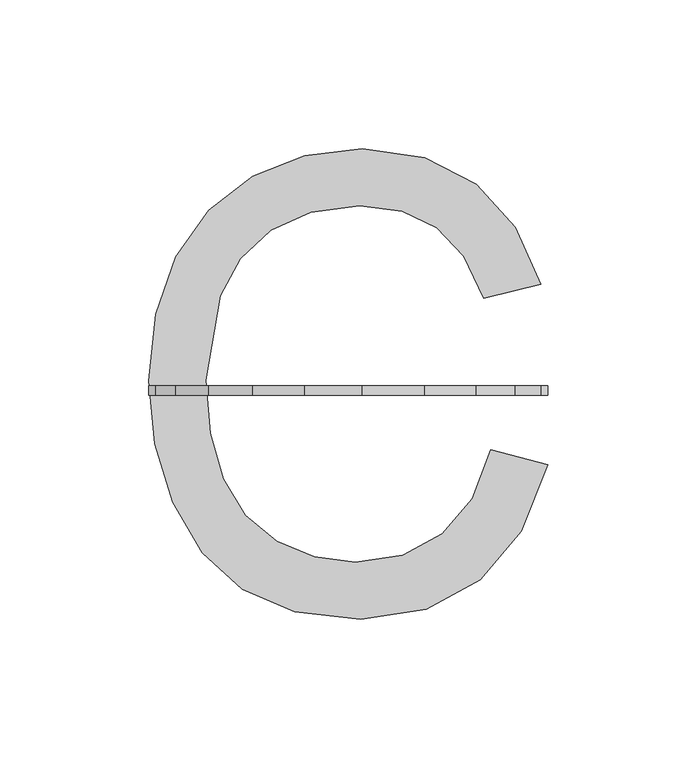
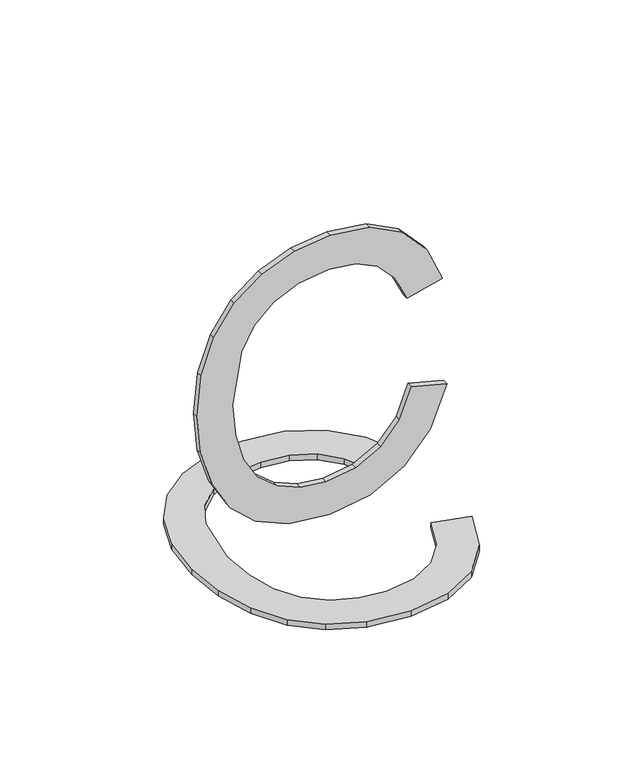
"""IFC4 building model written with IfcOpenShell, lengths in millimetres: proxy geometry, Grid Number1_FedEx : Grid Number1_FedEx."""

from ifc_helpers import new_model, si_unit, frame, origin, origin_with_axes, place, context, project, spatial, polyline, outline, extrude, source, transform, mapped, element, save


def entourage_191fb28f(model_context):
    return source(origin(), model_context, "Body", "SweptSolid", [
        extrude(outline(polyline([(-60.231609, 201.0047013), (-41.0946819, 196.0709623), (-49.9249535, 173.7710226), (-63.782406, 157.4794052), (-81.9849129, 147.5138131), (-103.8503471, 144.191949), (-126.0475006, 146.7055396), (-143.6753389, 154.2463111), (-157.187056, 166.552626), (-167.0358456, 183.3628467), (-173.0488401, 203.1258353), (-175.0531715, 224.2904544), (-172.7872024, 246.6137546), (-165.9892949, 265.8908447), (-155.0145289, 281.5096795), (-140.2179839, 292.8582136), (-122.6695713, 299.7682515), (-103.4392022, 302.0715975), (-82.4567951, 299.0907968), (-65.1092828, 290.1483949), (-51.9386292, 275.7956995), (-43.4867978, 256.5840188), (-62.6237249, 252.0240479), (-69.2581088, 265.9796146), (-78.3219854, 275.5527503), (-89.9274851, 281.0891904), (-104.1867384, 282.9346704), (-120.6231909, 280.88829), (-134.1255638, 274.7491488), (-144.371482, 265.1619969), (-151.0385706, 252.7715842), (-155.9162444, 224.3278312), (-154.4725651, 206.6485997), (-150.1415272, 191.3614842), (-142.7596071, 179.0504971), (-132.1632812, 170.2996513), (-119.4598377, 165.0715699), (-105.7565645, 163.3288761), (-89.78265, 165.7023036), (-76.4718333, 172.822586), (-66.4221433, 184.6149698), (-60.231609, 201.0047013)])), origin_with_axes(), (0.0, 0.0, 1.0), 3.175),
        extrude(outline(polyline([(68.9005296, -60.231609), (52.5107981, -66.4221433), (40.7184144, -76.4718333), (33.5981319, -89.78265), (31.2247044, -105.7565645), (32.9673982, -119.4598377), (38.1954796, -132.1632812), (46.9463254, -142.7596071), (59.2573125, -150.1415272), (74.5444281, -154.4725651), (92.2236595, -155.9162444), (120.6674125, -151.0385706), (133.0578252, -144.371482), (142.6449772, -134.1255638), (148.7841183, -120.6231909), (150.8304987, -104.1867384), (148.9850187, -89.9274851), (143.4485786, -78.3219854), (133.875443, -69.2581088), (119.9198763, -62.6237249), (124.4798472, -43.4867978), (143.6915279, -51.9386292), (158.0442232, -65.1092828), (166.9866251, -82.4567951), (169.9674258, -103.4392022), (167.6640798, -122.6695713), (160.754042, -140.2179839), (149.4055078, -155.0145289), (133.786673, -165.9892949), (114.5095829, -172.7872024), (92.1862827, -175.0531715), (71.0216636, -173.0488401), (51.258675, -167.0358456), (34.4484544, -157.187056), (22.1421394, -143.6753389), (14.6013679, -126.0475006), (12.0877774, -103.8503471), (15.4096414, -81.9849129), (25.3752336, -63.782406), (41.6668509, -49.9249535), (63.9667906, -41.0946819), (68.9005296, -60.231609)])), frame((0.0, 219.3456765, 0.0), z_axis=(0.0, 1.0, 0.0), x_axis=(0.0, 0.0, 1.0)), (0.0, 0.0, 1.0), 3.175),
    ])


if __name__ == "__main__":
    model = new_model("IFC4")
    model_context = context("Model", 3, world=origin())
    ifc_project = project(units=[si_unit("LENGTHUNIT", "METRE", prefix="MILLI")], contexts=[model_context])
    site = spatial("IfcSite", under=ifc_project)
    building = spatial("IfcBuilding", under=site)
    placement = place(None, origin())
    entourage_shape = entourage_191fb28f(model_context)
    element("IfcBuildingElementProxy", 1, Name="Grid Number1_FedEx : Grid Number1_FedEx", ObjectType="Grid Number1_FedEx : Grid Number1_FedEx", at=placement, inside=building, context=model_context, shape_type="MappedRepresentation", body=[
        mapped(entourage_shape, transform((0.0, 0.0, 0.0), x_axis=(1.0, 0.0, 0.0), y_axis=(0.0, 1.0, 0.0), z_axis=(0.0, 0.0, 1.0))),
    ])
    save(model, "model.ifc")

# Revit data of these elements
# Type "Grid Number1_FedEx : Grid Number1_FedEx"
#   Grid [instance default] = "S.8"
#   Label Width [instance default] = 1' - 0"
#   Half Box Width2 [instance default] = 0' - 6.13846"
#   Half Box Width [instance default] = 0' - 6"
#   Robust [instance default] = yes
#   Height = 0
#   Assembly Code = ""
# Element 1 (IfcBuildingElementProxy, "Grid Number1_FedEx : Grid Number1_FedEx")
#   Grid = "C"
#   Robust = no
#   Materials on its faces: "Letter"
# Materials
#   "Letter": class "Unassigned", colour RGB 178 187 30, transparency 0, Comments = "Rendering appearance not upgraded "
